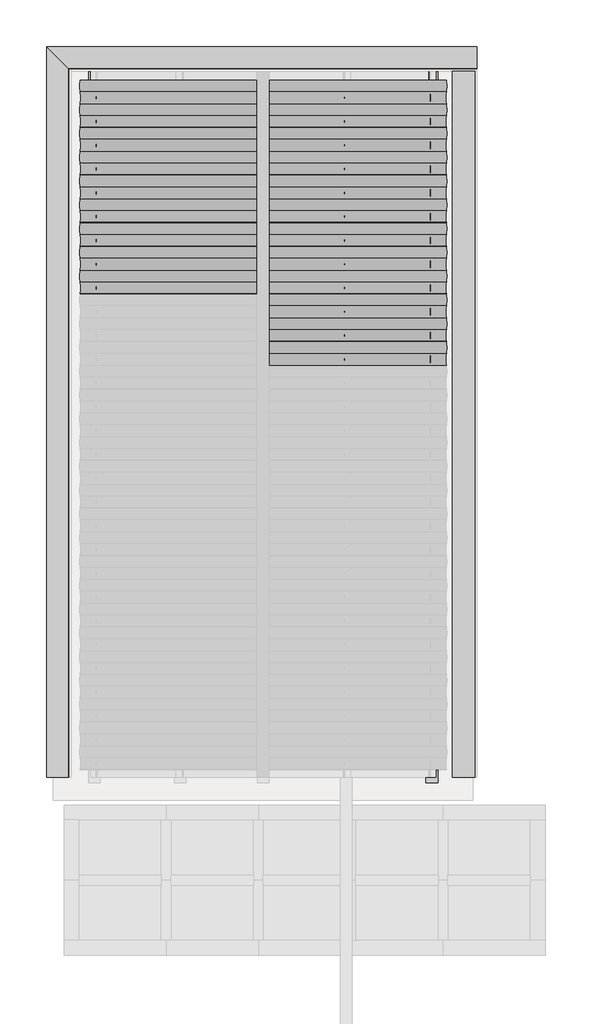
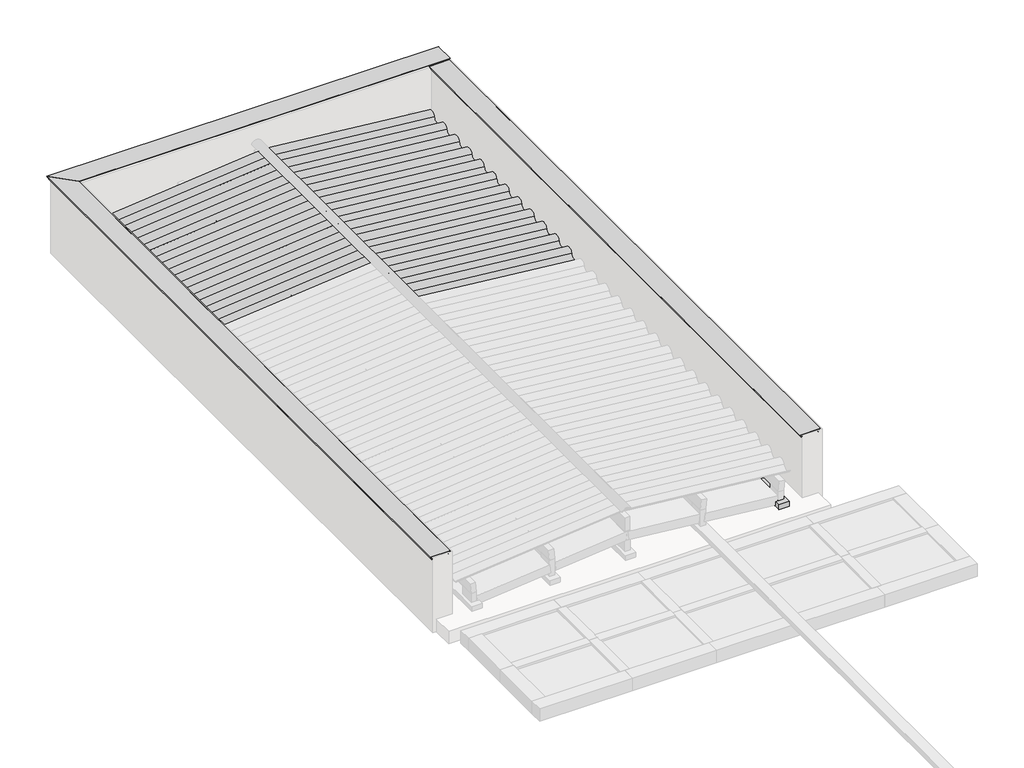
# One storey, part 3 of 3: 34 beams, 12 columns, 1 proxy.
"""IFC4 building model written with IfcOpenShell, lengths in millimetres."""

import ifcopenshell
import ifcopenshell.guid

model = None  # the IFC model being written
_history = None  # IfcOwnerHistory: only IFC2X3 demands one
_inside = {}  # id of a spatial element -> (the spatial element, [elements in it])
_under = {}  # id of a project, library or spatial element -> (it, [spatial elements below it])
_declared = {}  # id of a project -> (the project, [libraries it declares])
_typed = {}  # id of a type object -> (the type object, [elements of that type])
_made_of = {}  # id of a material, layer set ... -> (it, [elements and type objects made of it])


def new_model(schema):
    """Start an empty IFC model of exactly this schema.

    Asked for "IFC4X3", IfcOpenShell would pick the latest addendum, in which some entities
    have other attributes; the version numbers below select the first issue.
    IFC2X3 requires an IfcOwnerHistory on every rooted entity: one is made here for all.
    """
    global model, _history
    if schema == "IFC4X3":
        model = ifcopenshell.file(schema_version=(4, 3, 0, 0))
    else:
        model = ifcopenshell.file(schema=schema)
    _inside.clear()
    _under.clear()
    _declared.clear()
    _typed.clear()
    _made_of.clear()
    _history = None
    if model.schema == "IFC2X3":
        org = make("IfcOrganization", Name="unknown")
        user = make(
            "IfcPersonAndOrganization",
            ThePerson=make("IfcPerson", FamilyName="unknown"),
            TheOrganization=org,
        )
        app = make(
            "IfcApplication",
            ApplicationDeveloper=org,
            Version="unknown",
            ApplicationFullName="unknown",
            ApplicationIdentifier="unknown",
        )
        _history = make(
            "IfcOwnerHistory",
            OwningUser=user,
            OwningApplication=app,
            ChangeAction="ADDED",
            CreationDate=0,
        )
    return model


def make(cls, **values):
    """One entity of the class cls with the attributes given. An attribute that is None is left unset."""
    return model.create_entity(
        cls, **{name: value for name, value in values.items() if value is not None}
    )


def rooted(cls, **values):
    """An entity with a GlobalId (a new one), such as an element, a storey or a relation."""
    return make(cls, GlobalId=ifcopenshell.guid.new(), OwnerHistory=_history, **values)


def si_unit(unit_type, name, prefix=None):
    """IfcSIUnit, for example si_unit("LENGTHUNIT", "METRE", prefix="MILLI")."""
    return make("IfcSIUnit", UnitType=unit_type, Prefix=prefix, Name=name)


def assignment(units):
    """IfcUnitAssignment: the units of a project."""
    return None if units is None else make("IfcUnitAssignment", Units=units)


def point(xyz):
    """IfcCartesianPoint."""
    return None if xyz is None else make("IfcCartesianPoint", Coordinates=xyz)


def direction(xyz):
    """IfcDirection."""
    return None if xyz is None else make("IfcDirection", DirectionRatios=xyz)


def frame(location, z_axis=None, x_axis=None):
    """IfcAxis2Placement3D, a coordinate frame: its origin and axes. An axis left out is left unset."""
    return make(
        "IfcAxis2Placement3D",
        Location=point(location),
        Axis=direction(z_axis),
        RefDirection=direction(x_axis),
    )


def frame_2d(location, x_axis=None):
    """IfcAxis2Placement2D, a coordinate frame in the plane: its origin and x axis."""
    return make(
        "IfcAxis2Placement2D", Location=point(location), RefDirection=direction(x_axis)
    )


def origin():
    """The frame at (0, 0, 0) with its axes left unset."""
    return frame((0.0, 0.0, 0.0))


def place(relative_to, where):
    """IfcLocalPlacement: puts the frame where relative to a parent placement (None: the world)."""
    return make(
        "IfcLocalPlacement", PlacementRelTo=relative_to, RelativePlacement=where
    )


def context(
    kind, dimensions, precision=None, world=None, true_north=None, identifier=None
):
    """IfcGeometricRepresentationContext, for example the 3D "Model" context."""
    return make(
        "IfcGeometricRepresentationContext",
        ContextIdentifier=identifier,
        ContextType=kind,
        CoordinateSpaceDimension=dimensions,
        Precision=precision,
        WorldCoordinateSystem=world,
        TrueNorth=true_north,
    )


def project(units=None, contexts=None):
    """IfcProject with its units and contexts."""
    return rooted(
        "IfcProject",
        Name="project",
        RepresentationContexts=contexts,
        UnitsInContext=assignment(units),
    )


def spatial(cls, under=None, at=None, **own):
    """A site, building, storey or space (cls), placed at a placement, below another one or the project."""
    s = rooted(cls, ObjectPlacement=at, **own)
    if under is not None:
        _under.setdefault(under.id(), (under, []))[1].append(s)
    return s


def polyline(points):
    """IfcPolyline through the points."""
    return make("IfcPolyline", Points=[point(p) for p in points])


def circle_curve(where, radius):
    """IfcCircle in the frame where."""
    return make("IfcCircle", Position=where, Radius=radius)


def trimmed(basis, trim1, trim2, sense, master):
    """IfcTrimmedCurve: the piece of a basis curve between two trims."""
    return make(
        "IfcTrimmedCurve",
        BasisCurve=basis,
        Trim1=trim1,
        Trim2=trim2,
        SenseAgreement=sense,
        MasterRepresentation=master,
    )


def segment(curve, same_sense, transition):
    """IfcCompositeCurveSegment."""
    return make(
        "IfcCompositeCurveSegment",
        Transition=transition,
        SameSense=same_sense,
        ParentCurve=curve,
    )


def composite_curve(segments, self_intersect=None):
    """IfcCompositeCurve: segments joined end to end."""
    return make("IfcCompositeCurve", Segments=segments, SelfIntersect=self_intersect)


def outline(outer, holes=None, kind="AREA"):
    """IfcArbitraryClosedProfileDef: a profile drawn as a closed curve; with holes, ...WithVoids."""
    if holes is None:
        return make("IfcArbitraryClosedProfileDef", ProfileType=kind, OuterCurve=outer)
    return make(
        "IfcArbitraryProfileDefWithVoids",
        ProfileType=kind,
        OuterCurve=outer,
        InnerCurves=holes,
    )


def extrude(swept, where, along, depth):
    """IfcExtrudedAreaSolid: the profile swept, set in the frame where, extruded along a direction by depth."""
    return make(
        "IfcExtrudedAreaSolid",
        SweptArea=swept,
        Position=where,
        ExtrudedDirection=direction(along),
        Depth=depth,
    )


def faces_of(points, faces, orient=None, outer=None):
    """IfcFace entities. A face is a list of loops; a loop is a list of indices into points, from 0.

    orient and outer hold one flag for each loop. By default every Orientation is true, the
    first loop of a face is its IfcFaceOuterBound and the others are IfcFaceBound.
    """
    made = []
    for i, loops in enumerate(faces):
        bounds = []
        for j, loop in enumerate(loops):
            is_outer = j == 0 if outer is None else outer[i][j]
            bounds.append(
                make(
                    "IfcFaceOuterBound" if is_outer else "IfcFaceBound",
                    Bound=make("IfcPolyLoop", Polygon=[points[k] for k in loop]),
                    Orientation=True if orient is None else orient[i][j],
                )
            )
        made.append(make("IfcFace", Bounds=bounds))
    return made


def faceted_brep(points, faces, orient=None, outer=None, voids=None):
    """IfcFacetedBrep: a solid bounded by flat faces; with voids (closed shells), ...WithVoids."""
    shared = [point(p) for p in points]
    hull = make("IfcClosedShell", CfsFaces=faces_of(shared, faces, orient, outer))
    if voids is None:
        return make("IfcFacetedBrep", Outer=hull)
    return make(
        "IfcFacetedBrepWithVoids",
        Outer=hull,
        Voids=[
            make(cls, CfsFaces=faces_of(shared, fs, o, b)) for cls, fs, o, b in voids
        ],
    )


def shape(context_of_items, identifier, shape_type, items):
    """IfcShapeRepresentation: the items that make up one representation, for example the "Body"."""
    return make(
        "IfcShapeRepresentation",
        ContextOfItems=context_of_items,
        RepresentationIdentifier=identifier,
        RepresentationType=shape_type,
        Items=items,
    )


def source(mapping_origin, context_of_items, identifier, shape_type, items):
    """IfcRepresentationMap: a shape defined once, which mapped items show again and again."""
    return make(
        "IfcRepresentationMap",
        MappingOrigin=mapping_origin,
        MappedRepresentation=shape(context_of_items, identifier, shape_type, items),
    )


def transform(
    local_origin,
    x_axis=None,
    y_axis=None,
    z_axis=None,
    scale=None,
    scale2=None,
    scale3=None,
    uniform=True,
):
    """IfcCartesianTransformationOperator3D, or its non-uniform kind. x_axis, y_axis, z_axis: its Axis1, 2, 3."""
    if uniform:
        return make(
            "IfcCartesianTransformationOperator3D",
            Axis1=direction(x_axis),
            Axis2=direction(y_axis),
            LocalOrigin=point(local_origin),
            Scale=scale,
            Axis3=direction(z_axis),
        )
    return make(
        "IfcCartesianTransformationOperator3DnonUniform",
        Axis1=direction(x_axis),
        Axis2=direction(y_axis),
        LocalOrigin=point(local_origin),
        Scale=scale,
        Axis3=direction(z_axis),
        Scale2=scale2,
        Scale3=scale3,
    )


def mapped(mapping_source, mapping_target):
    """IfcMappedItem: shows the shape of a source again, moved by a transform."""
    return make(
        "IfcMappedItem", MappingSource=mapping_source, MappingTarget=mapping_target
    )


def made_of(thing, what):
    """Note that an element or type object is made of a material, layer set ...; save() writes the relation."""
    if what is not None:
        _made_of.setdefault(what.id(), (what, []))[1].append(thing)
    return thing


def element(
    cls,
    number,
    at=None,
    inside=None,
    cuts=None,
    type_object=None,
    material=None,
    context=None,
    identifier="Body",
    shape_type=None,
    held_by="IfcProductDefinitionShape",
    body=None,
    shapes=None,
    **own,
):
    """One element of the class cls, such as IfcWall. Its Tag is "e" and its number.

    at: its placement. inside: the storey or other place that contains it. cuts: it is an
    opening in that element (IfcRelVoidsElement). A single representation is given by context,
    identifier, shape_type and body (its items); several are given by shapes. held_by: the class
    of the entity that holds the representations. save() writes the other relations.
    """
    e = rooted(cls, Tag="e%d" % number, ObjectPlacement=at, **own)
    if body is not None:
        shapes = [shape(context, identifier, shape_type, body)]
    if shapes is not None:
        e.Representation = make(held_by, Representations=shapes)
    if inside is not None:
        _inside.setdefault(inside.id(), (inside, []))[1].append(e)
    if cuts is not None:
        rooted(
            "IfcRelVoidsElement", RelatingBuildingElement=cuts, RelatedOpeningElement=e
        )
    if type_object is not None:
        _typed.setdefault(type_object.id(), (type_object, []))[1].append(e)
    return made_of(e, material)


def aggregate(whole, parts):
    """IfcRelAggregates: a whole, such as a stair, and the parts it consists of."""
    return rooted("IfcRelAggregates", RelatingObject=whole, RelatedObjects=parts)


def save(model, path):
    """Write the relations noted so far, then the file.

    IfcRelAggregates (storeys below a building ...), IfcRelContainedInSpatialStructure (elements
    in a storey), IfcRelDefinesByType, IfcRelAssociatesMaterial and IfcRelDeclares: one each for
    every whole, place, type object, material and project.
    """
    for whole, parts in _under.values():
        aggregate(whole, parts)
    for where, things in _inside.values():
        rooted(
            "IfcRelContainedInSpatialStructure",
            RelatedElements=things,
            RelatingStructure=where,
        )
    for kind, things in _typed.values():
        rooted("IfcRelDefinesByType", RelatedObjects=things, RelatingType=kind)
    for what, things in _made_of.values():
        rooted("IfcRelAssociatesMaterial", RelatedObjects=things, RelatingMaterial=what)
    for by, libraries in _declared.values():
        rooted("IfcRelDeclares", RelatingContext=by, RelatedDefinitions=libraries)
    model.write(path)


def column_1cffec27(model_context):
    return source(origin(), model_context, "Body", "SweptSolid", [
        extrude(outline(polyline([(30.0, 80.0), (30.0, -80.0), (-30.0, -80.0), (-30.0, 80.0), (30.0, 80.0)])), frame((0.0, 0.0, 3110.0), z_axis=(0.0, 0.0, 1.0), x_axis=(1.0, 0.0, 0.0)), (0.0, 0.0, 1.0), 238.0),
    ])


def column_35730ad5(model_context):
    return source(origin(), model_context, "Body", "SweptSolid", [
        extrude(outline(polyline([(30.0, 80.0), (30.0, -80.0), (-30.0, -80.0), (-30.0, 80.0), (30.0, 80.0)])), frame((0.0, 0.0, 3110.0), z_axis=(0.0, 0.0, 1.0), x_axis=(1.0, 0.0, 0.0)), (0.0, 0.0, 1.0), 197.9),
    ])


def column_00c463e4(model_context):
    return source(origin(), model_context, "Body", "SweptSolid", [
        extrude(outline(polyline([(30.0, 80.0), (30.0, -80.0), (-30.0, -80.0), (-30.0, 80.0), (30.0, 80.0)])), frame((0.0, 0.0, 3110.0), z_axis=(0.0, 0.0, 1.0), x_axis=(1.0, 0.0, 0.0)), (0.0, 0.0, 1.0), 109.8),
    ])


model = new_model("IFC4")

# Units and contexts
model_context = context("Model", 3, world=origin())
ifc_project = project(units=[si_unit("LENGTHUNIT", "METRE", prefix="MILLI")], contexts=[model_context])

# Site, building, storey
site = spatial("IfcSite", under=ifc_project)
building = spatial("IfcBuilding", under=site)
storey = spatial("IfcBuildingStorey", under=building, Name="COB. GARAGEM", Elevation=3050.0)

# Beams
placement = place(None, origin())
element("IfcBeam", 1, ObjectType="Madeira de lei : Berço 6x12cm", at=placement, inside=storey, context=model_context, shape_type="SweptSolid", body=[
    extrude(outline(polyline([(-9620.281307, 6423.9300153), (-9500.281307, 6423.9300153), (-9500.281307, 4423.9300153), (-9620.281307, 4423.9300153), (-9620.281307, 6423.9300153)])), frame((0.0, 0.0, 3050.0), z_axis=(0.0, 0.0, 1.0), x_axis=(1.0, 0.0, 0.0)), (0.0, 0.0, 1.0), 60.0),
])
element("IfcBeam", 2, ObjectType="Madeira de lei : Berço 6x12cm", at=placement, inside=storey, context=model_context, shape_type="SweptSolid", body=[
    extrude(outline(polyline([(-9620.281307, 7083.9300153), (-9500.281307, 7083.9300153), (-9500.281307, 6423.9300153), (-9620.281307, 6423.9300153), (-9620.281307, 7083.9300153)])), frame((0.0, 0.0, 3050.0), z_axis=(0.0, 0.0, 1.0), x_axis=(1.0, 0.0, 0.0)), (0.0, 0.0, 1.0), 60.0),
])
element("IfcBeam", 3, ObjectType="Madeira de lei : Berço 6x12cm", at=placement, inside=storey, context=model_context, shape_type="SweptSolid", body=[
    extrude(outline(polyline([(-8767.0824227, 6423.9300153), (-8647.0824227, 6423.9300153), (-8647.0824227, 4423.9300153), (-8767.0824227, 4423.9300153), (-8767.0824227, 6423.9300153)])), frame((0.0, 0.0, 3050.0), z_axis=(0.0, 0.0, 1.0), x_axis=(1.0, 0.0, 0.0)), (0.0, 0.0, 1.0), 60.0),
])
element("IfcBeam", 4, ObjectType="Madeira de lei : Berço 6x12cm", at=placement, inside=storey, context=model_context, shape_type="SweptSolid", body=[
    extrude(outline(polyline([(-8767.0824227, 7083.9300153), (-8647.0824227, 7083.9300153), (-8647.0824227, 6423.9300153), (-8767.0824227, 6423.9300153), (-8767.0824227, 7083.9300153)])), frame((0.0, 0.0, 3050.0), z_axis=(0.0, 0.0, 1.0), x_axis=(1.0, 0.0, 0.0)), (0.0, 0.0, 1.0), 60.0),
])
element("IfcBeam", 5, ObjectType="Madeira de lei : Berço 6x12cm", at=placement, inside=storey, context=model_context, shape_type="SweptSolid", body=[
    extrude(outline(polyline([(-7884.0324227, 4423.9300153), (-7764.0324227, 4423.9300153), (-7764.0324227, 2423.9300153), (-7884.0324227, 2423.9300153), (-7884.0324227, 4423.9300153)])), frame((0.0, 0.0, 3050.0), z_axis=(0.0, 0.0, 1.0), x_axis=(1.0, 0.0, 0.0)), (0.0, 0.0, 1.0), 60.0),
])
element("IfcBeam", 6, ObjectType="Madeira de lei : Berço 6x12cm", at=placement, inside=storey, context=model_context, shape_type="SweptSolid", body=[
    extrude(outline(polyline([(-7884.0324227, 6423.9300153), (-7764.0324227, 6423.9300153), (-7764.0324227, 4423.9300153), (-7884.0324227, 4423.9300153), (-7884.0324227, 6423.9300153)])), frame((0.0, 0.0, 3050.0), z_axis=(0.0, 0.0, 1.0), x_axis=(1.0, 0.0, 0.0)), (0.0, 0.0, 1.0), 60.0),
])
element("IfcBeam", 7, ObjectType="Madeira de lei : Berço 6x12cm", at=placement, inside=storey, context=model_context, shape_type="SweptSolid", body=[
    extrude(outline(polyline([(-7884.0324227, 2423.9300153), (-7764.0324227, 2423.9300153), (-7764.0324227, 423.9300153), (-7884.0324227, 423.9300153), (-7884.0324227, 2423.9300153)])), frame((0.0, 0.0, 3050.0), z_axis=(0.0, 0.0, 1.0), x_axis=(1.0, 0.0, 0.0)), (0.0, 0.0, 1.0), 60.0),
])
element("IfcBeam", 8, ObjectType="Madeira de lei : Berço 6x12cm", at=placement, inside=storey, context=model_context, shape_type="SweptSolid", body=[
    extrude(outline(polyline([(-7884.0324227, 7083.9300153), (-7764.0324227, 7083.9300153), (-7764.0324227, 6423.9300153), (-7884.0324227, 6423.9300153), (-7884.0324227, 7083.9300153)])), frame((0.0, 0.0, 3050.0), z_axis=(0.0, 0.0, 1.0), x_axis=(1.0, 0.0, 0.0)), (0.0, 0.0, 1.0), 60.0),
])
element("IfcBeam", 9, ObjectType="Madeira de lei : Berço 6x12cm", at=placement, inside=storey, context=model_context, shape_type="SweptSolid", body=[
    extrude(outline(polyline([(-7884.0324227, 423.9300153), (-7764.0324227, 423.9300153), (-7764.0324227, -236.0699847), (-7884.0324227, -236.0699847), (-7884.0324227, 423.9300153)])), frame((0.0, 0.0, 3050.0), z_axis=(0.0, 0.0, 1.0), x_axis=(1.0, 0.0, 0.0)), (0.0, 0.0, 1.0), 60.0),
])
element("IfcBeam", 10, ObjectType="Madeira de lei : Berço 6x12cm", at=placement, inside=storey, context=model_context, shape_type="SweptSolid", body=[
    extrude(outline(polyline([(-10473.4801913, 6423.9300153), (-10353.4801913, 6423.9300153), (-10353.4801913, 4423.9300153), (-10473.4801913, 4423.9300153), (-10473.4801913, 6423.9300153)])), frame((0.0, 0.0, 3050.0), z_axis=(0.0, 0.0, 1.0), x_axis=(1.0, 0.0, 0.0)), (0.0, 0.0, 1.0), 60.0),
])
element("IfcBeam", 11, ObjectType="Madeira de lei : Berço 6x12cm", at=placement, inside=storey, context=model_context, shape_type="SweptSolid", body=[
    extrude(outline(polyline([(-10473.4801913, 7083.9300153), (-10353.4801913, 7083.9300153), (-10353.4801913, 6423.9300153), (-10473.4801913, 6423.9300153), (-10473.4801913, 7083.9300153)])), frame((0.0, 0.0, 3050.0), z_axis=(0.0, 0.0, 1.0), x_axis=(1.0, 0.0, 0.0)), (0.0, 0.0, 1.0), 60.0),
])
element("IfcBeam", 12, ObjectType="Madeira de lei : Berço 6x12cm", at=placement, inside=storey, context=model_context, shape_type="SweptSolid", body=[
    extrude(outline(polyline([(-11356.5301913, 6423.9300153), (-11236.5301913, 6423.9300153), (-11236.5301913, 4423.9300153), (-11356.5301913, 4423.9300153), (-11356.5301913, 6423.9300153)])), frame((0.0, 0.0, 3050.0), z_axis=(0.0, 0.0, 1.0), x_axis=(1.0, 0.0, 0.0)), (0.0, 0.0, 1.0), 60.0),
])
element("IfcBeam", 13, ObjectType="Madeira de lei : Berço 6x12cm", at=placement, inside=storey, context=model_context, shape_type="SweptSolid", body=[
    extrude(outline(polyline([(-11356.5301913, 7083.9300153), (-11236.5301913, 7083.9300153), (-11236.5301913, 6423.9300153), (-11356.5301913, 6423.9300153), (-11356.5301913, 7083.9300153)])), frame((0.0, 0.0, 3050.0), z_axis=(0.0, 0.0, 1.0), x_axis=(1.0, 0.0, 0.0)), (0.0, 0.0, 1.0), 60.0),
])
element("IfcBeam", 14, ObjectType="Telha Ondulada : Fibrocimento", at=placement, inside=storey, context=model_context, shape_type="SweptSolid", body=[
    extrude(outline(composite_curve([segment(trimmed(circle_curve(frame_2d((-58.7002979, -53.2060538)), 66.7939461), [point((-29.350149, 6.7939462))], [point((-29.350149, -113.2060538))], False, "CARTESIAN"), True, "CONTINUOUS"), segment(polyline([(-29.350149, -113.2060538), (-31.5472155, -108.7146288)]), True, "CONTINUOUS"), segment(trimmed(circle_curve(frame_2d((-58.7002979, -53.2060538)), 61.7939461), [point((-31.5472155, -108.7146288))], [point((-31.5472155, 2.3025211))], True, "CARTESIAN"), True, "CONTINUOUS"), segment(trimmed(circle_curve(frame_2d((0.0, 66.7939462)), 71.7939461), [point((-31.5472155, 2.3025211))], [point((-31.5472155, 131.2853712))], False, "CARTESIAN"), True, "CONTINUOUS"), segment(polyline([(-31.5472155, 131.2853712), (-29.350149, 126.7939462)]), True, "CONTINUOUS"), segment(trimmed(circle_curve(frame_2d((0.0, 66.7939462)), 66.7939461), [point((-29.350149, 126.7939462))], [point((-29.350149, 6.7939462))], True, "CARTESIAN"), True, "CONTINUOUS")], self_intersect=False)), frame((-11446.918865, 4918.826948, 3394.3067746), z_axis=(0.9950371902099892, 0.0, 0.09950371902099903), x_axis=(-0.09950371902099903, 0.0, 0.9950371902099892)), (0.0, 0.0, 1.0), 1886.8678854),
])
element("IfcBeam", 15, ObjectType="Telha Ondulada : Fibrocimento", at=placement, inside=storey, context=model_context, shape_type="SweptSolid", body=[
    extrude(outline(composite_curve([segment(trimmed(circle_curve(frame_2d((-58.7002979, -53.2060538)), 66.7939461), [point((-29.350149, 6.7939462))], [point((-29.350149, -113.2060538))], False, "CARTESIAN"), True, "CONTINUOUS"), segment(polyline([(-29.350149, -113.2060538), (-31.5472155, -108.7146288)]), True, "CONTINUOUS"), segment(trimmed(circle_curve(frame_2d((-58.7002979, -53.2060538)), 61.7939461), [point((-31.5472155, -108.7146288))], [point((-31.5472155, 2.3025211))], True, "CARTESIAN"), True, "CONTINUOUS"), segment(trimmed(circle_curve(frame_2d((0.0, 66.7939462)), 71.7939461), [point((-31.5472155, 2.3025211))], [point((-31.5472155, 131.2853712))], False, "CARTESIAN"), True, "CONTINUOUS"), segment(polyline([(-31.5472155, 131.2853712), (-29.350149, 126.7939462)]), True, "CONTINUOUS"), segment(trimmed(circle_curve(frame_2d((0.0, 66.7939462)), 66.7939461), [point((-29.350149, 126.7939462))], [point((-29.350149, 6.7939462))], True, "CARTESIAN"), True, "CONTINUOUS")], self_intersect=False)), frame((-11446.918865, 5163.326948, 3394.3067746), z_axis=(0.9950371902099892, 0.0, 0.09950371902099937), x_axis=(-0.09950371902099937, 0.0, 0.9950371902099892)), (0.0, 0.0, 1.0), 1886.8678854),
])
element("IfcBeam", 16, ObjectType="Telha Ondulada : Fibrocimento", at=placement, inside=storey, context=model_context, shape_type="SweptSolid", body=[
    extrude(outline(composite_curve([segment(trimmed(circle_curve(frame_2d((-58.7002979, -53.2060538)), 66.7939461), [point((-29.350149, 6.7939462))], [point((-29.350149, -113.2060538))], False, "CARTESIAN"), True, "CONTINUOUS"), segment(polyline([(-29.350149, -113.2060538), (-31.5472155, -108.7146288)]), True, "CONTINUOUS"), segment(trimmed(circle_curve(frame_2d((-58.7002979, -53.2060538)), 61.7939461), [point((-31.5472155, -108.7146288))], [point((-31.5472155, 2.3025211))], True, "CARTESIAN"), True, "CONTINUOUS"), segment(trimmed(circle_curve(frame_2d((0.0, 66.7939462)), 71.7939461), [point((-31.5472155, 2.3025211))], [point((-31.5472155, 131.2853712))], False, "CARTESIAN"), True, "CONTINUOUS"), segment(polyline([(-31.5472155, 131.2853712), (-29.350149, 126.7939462)]), True, "CONTINUOUS"), segment(trimmed(circle_curve(frame_2d((0.0, 66.7939462)), 66.7939461), [point((-29.350149, 126.7939462))], [point((-29.350149, 6.7939462))], True, "CARTESIAN"), True, "CONTINUOUS")], self_intersect=False)), frame((-11446.918865, 5407.826948, 3394.3067746), z_axis=(0.9950371902099892, 0.0, 0.09950371902099972), x_axis=(-0.09950371902099972, 0.0, 0.9950371902099892)), (0.0, 0.0, 1.0), 1886.8678854),
])
element("IfcBeam", 17, ObjectType="Telha Ondulada : Fibrocimento", at=placement, inside=storey, context=model_context, shape_type="SweptSolid", body=[
    extrude(outline(composite_curve([segment(trimmed(circle_curve(frame_2d((-58.7002979, -53.2060538)), 66.7939461), [point((-29.350149, 6.7939462))], [point((-29.350149, -113.2060538))], False, "CARTESIAN"), True, "CONTINUOUS"), segment(polyline([(-29.350149, -113.2060538), (-31.5472155, -108.7146288)]), True, "CONTINUOUS"), segment(trimmed(circle_curve(frame_2d((-58.7002979, -53.2060538)), 61.7939461), [point((-31.5472155, -108.7146288))], [point((-31.5472155, 2.3025211))], True, "CARTESIAN"), True, "CONTINUOUS"), segment(trimmed(circle_curve(frame_2d((0.0, 66.7939462)), 71.7939461), [point((-31.5472155, 2.3025211))], [point((-31.5472155, 131.2853712))], False, "CARTESIAN"), True, "CONTINUOUS"), segment(polyline([(-31.5472155, 131.2853712), (-29.350149, 126.7939462)]), True, "CONTINUOUS"), segment(trimmed(circle_curve(frame_2d((0.0, 66.7939462)), 66.7939461), [point((-29.350149, 126.7939462))], [point((-29.350149, 6.7939462))], True, "CARTESIAN"), True, "CONTINUOUS")], self_intersect=False)), frame((-11446.918865, 5652.326948, 3394.3067746), z_axis=(0.9950371902099892, 0.0, 0.09950371902099954), x_axis=(-0.09950371902099954, 0.0, 0.9950371902099892)), (0.0, 0.0, 1.0), 1886.8678854),
])
element("IfcBeam", 18, ObjectType="Telha Ondulada : Fibrocimento", at=placement, inside=storey, context=model_context, shape_type="SweptSolid", body=[
    extrude(outline(composite_curve([segment(trimmed(circle_curve(frame_2d((-58.7002979, -53.2060538)), 66.7939461), [point((-29.350149, 6.7939462))], [point((-29.350149, -113.2060538))], False, "CARTESIAN"), True, "CONTINUOUS"), segment(polyline([(-29.350149, -113.2060538), (-31.5472155, -108.7146288)]), True, "CONTINUOUS"), segment(trimmed(circle_curve(frame_2d((-58.7002979, -53.2060538)), 61.7939461), [point((-31.5472155, -108.7146288))], [point((-31.5472155, 2.3025211))], True, "CARTESIAN"), True, "CONTINUOUS"), segment(trimmed(circle_curve(frame_2d((0.0, 66.7939462)), 71.7939461), [point((-31.5472155, 2.3025211))], [point((-31.5472155, 131.2853712))], False, "CARTESIAN"), True, "CONTINUOUS"), segment(polyline([(-31.5472155, 131.2853712), (-29.350149, 126.7939462)]), True, "CONTINUOUS"), segment(trimmed(circle_curve(frame_2d((0.0, 66.7939462)), 66.7939461), [point((-29.350149, 126.7939462))], [point((-29.350149, 6.7939462))], True, "CARTESIAN"), True, "CONTINUOUS")], self_intersect=False)), frame((-11446.918865, 5896.826948, 3394.3067746), z_axis=(0.9950371902099892, 0.0, 0.09950371902099932), x_axis=(-0.09950371902099932, 0.0, 0.9950371902099892)), (0.0, 0.0, 1.0), 1886.8678854),
])
element("IfcBeam", 19, ObjectType="Telha Ondulada : Fibrocimento", at=placement, inside=storey, context=model_context, shape_type="SweptSolid", body=[
    extrude(outline(composite_curve([segment(trimmed(circle_curve(frame_2d((-58.7002979, -53.2060538)), 66.7939461), [point((-29.350149, 6.7939462))], [point((-29.350149, -113.2060538))], False, "CARTESIAN"), True, "CONTINUOUS"), segment(polyline([(-29.350149, -113.2060538), (-31.5472155, -108.7146288)]), True, "CONTINUOUS"), segment(trimmed(circle_curve(frame_2d((-58.7002979, -53.2060538)), 61.7939461), [point((-31.5472155, -108.7146288))], [point((-31.5472155, 2.3025211))], True, "CARTESIAN"), True, "CONTINUOUS"), segment(trimmed(circle_curve(frame_2d((0.0, 66.7939462)), 71.7939461), [point((-31.5472155, 2.3025211))], [point((-31.5472155, 131.2853712))], False, "CARTESIAN"), True, "CONTINUOUS"), segment(polyline([(-31.5472155, 131.2853712), (-29.350149, 126.7939462)]), True, "CONTINUOUS"), segment(trimmed(circle_curve(frame_2d((0.0, 66.7939462)), 66.7939461), [point((-29.350149, 126.7939462))], [point((-29.350149, 6.7939462))], True, "CARTESIAN"), True, "CONTINUOUS")], self_intersect=False)), frame((-11446.918865, 6141.326948, 3394.3067746), z_axis=(0.9950371902099892, 0.0, 0.09950371902099943), x_axis=(-0.09950371902099943, 0.0, 0.9950371902099892)), (0.0, 0.0, 1.0), 1886.8678854),
])
element("IfcBeam", 20, ObjectType="Telha Ondulada : Fibrocimento", at=placement, inside=storey, context=model_context, shape_type="SweptSolid", body=[
    extrude(outline(composite_curve([segment(trimmed(circle_curve(frame_2d((-58.7002979, -53.2060538)), 66.7939461), [point((-29.350149, 6.7939462))], [point((-29.350149, -113.2060538))], False, "CARTESIAN"), True, "CONTINUOUS"), segment(polyline([(-29.350149, -113.2060538), (-31.5472155, -108.7146288)]), True, "CONTINUOUS"), segment(trimmed(circle_curve(frame_2d((-58.7002979, -53.2060538)), 61.7939461), [point((-31.5472155, -108.7146288))], [point((-31.5472155, 2.3025211))], True, "CARTESIAN"), True, "CONTINUOUS"), segment(trimmed(circle_curve(frame_2d((0.0, 66.7939462)), 71.7939461), [point((-31.5472155, 2.3025211))], [point((-31.5472155, 131.2853712))], False, "CARTESIAN"), True, "CONTINUOUS"), segment(polyline([(-31.5472155, 131.2853712), (-29.350149, 126.7939462)]), True, "CONTINUOUS"), segment(trimmed(circle_curve(frame_2d((0.0, 66.7939462)), 66.7939461), [point((-29.350149, 126.7939462))], [point((-29.350149, 6.7939462))], True, "CARTESIAN"), True, "CONTINUOUS")], self_intersect=False)), frame((-11446.918865, 6385.826948, 3394.3067746), z_axis=(0.9950371902099892, 0.0, 0.09950371902099919), x_axis=(-0.09950371902099919, 0.0, 0.9950371902099892)), (0.0, 0.0, 1.0), 1886.8678854),
])
element("IfcBeam", 21, ObjectType="Telha Ondulada : Fibrocimento", at=placement, inside=storey, context=model_context, shape_type="SweptSolid", body=[
    extrude(outline(composite_curve([segment(trimmed(circle_curve(frame_2d((-58.7002979, -53.2060538)), 66.7939461), [point((-29.350149, 6.7939462))], [point((-29.350149, -113.2060538))], False, "CARTESIAN"), True, "CONTINUOUS"), segment(polyline([(-29.350149, -113.2060538), (-31.5472155, -108.7146288)]), True, "CONTINUOUS"), segment(trimmed(circle_curve(frame_2d((-58.7002979, -53.2060538)), 61.7939461), [point((-31.5472155, -108.7146288))], [point((-31.5472155, 2.3025211))], True, "CARTESIAN"), True, "CONTINUOUS"), segment(trimmed(circle_curve(frame_2d((0.0, 66.7939462)), 71.7939461), [point((-31.5472155, 2.3025211))], [point((-31.5472155, 131.2853712))], False, "CARTESIAN"), True, "CONTINUOUS"), segment(polyline([(-31.5472155, 131.2853712), (-29.350149, 126.7939462)]), True, "CONTINUOUS"), segment(trimmed(circle_curve(frame_2d((0.0, 66.7939462)), 66.7939461), [point((-29.350149, 126.7939462))], [point((-29.350149, 6.7939462))], True, "CARTESIAN"), True, "CONTINUOUS")], self_intersect=False)), frame((-11446.918865, 6630.326948, 3394.3067746), z_axis=(0.9950371902099892, 0.0, 0.09950371902099925), x_axis=(-0.09950371902099925, 0.0, 0.9950371902099892)), (0.0, 0.0, 1.0), 1886.8678854),
])
element("IfcBeam", 22, ObjectType="Telha Ondulada : Fibrocimento", at=placement, inside=storey, context=model_context, shape_type="SweptSolid", body=[
    extrude(outline(composite_curve([segment(trimmed(circle_curve(frame_2d((-58.7002979, -53.2060538)), 66.7939461), [point((-29.350149, 6.7939462))], [point((-29.350149, -113.2060538))], False, "CARTESIAN"), True, "CONTINUOUS"), segment(polyline([(-29.350149, -113.2060538), (-31.5472155, -108.7146288)]), True, "CONTINUOUS"), segment(trimmed(circle_curve(frame_2d((-58.7002979, -53.2060538)), 61.7939461), [point((-31.5472155, -108.7146288))], [point((-31.5472155, 2.3025211))], True, "CARTESIAN"), True, "CONTINUOUS"), segment(trimmed(circle_curve(frame_2d((0.0, 66.7939462)), 71.7939461), [point((-31.5472155, 2.3025211))], [point((-31.5472155, 131.2853712))], False, "CARTESIAN"), True, "CONTINUOUS"), segment(polyline([(-31.5472155, 131.2853712), (-29.350149, 126.7939462)]), True, "CONTINUOUS"), segment(trimmed(circle_curve(frame_2d((0.0, 66.7939462)), 66.7939461), [point((-29.350149, 126.7939462))], [point((-29.350149, 6.7939462))], True, "CARTESIAN"), True, "CONTINUOUS")], self_intersect=False)), frame((-11446.918865, 6874.826948, 3394.3067746), z_axis=(0.9950371902099892, 0.0, 0.09950371902099937), x_axis=(-0.09950371902099937, 0.0, 0.9950371902099892)), (0.0, 0.0, 1.0), 1886.8678854),
])
element("IfcBeam", 23, ObjectType="Telha Ondulada : Fibrocimento", at=placement, inside=storey, context=model_context, shape_type="SweptSolid", body=[
    extrude(outline(composite_curve([segment(trimmed(circle_curve(frame_2d((0.0, 66.7939462)), 66.7939461), [point((29.350149, 6.7939462))], [point((29.350149, 126.7939462))], True, "CARTESIAN"), True, "CONTINUOUS"), segment(polyline([(29.350149, 126.7939462), (31.5472155, 131.2853712)]), True, "CONTINUOUS"), segment(trimmed(circle_curve(frame_2d((0.0, 66.7939462)), 71.7939461), [point((31.5472155, 131.2853712))], [point((31.5472155, 2.3025211))], False, "CARTESIAN"), True, "CONTINUOUS"), segment(trimmed(circle_curve(frame_2d((58.7002979, -53.2060538)), 61.7939461), [point((31.5472155, 2.3025211))], [point((31.5472155, -108.7146288))], True, "CARTESIAN"), True, "CONTINUOUS"), segment(polyline([(31.5472155, -108.7146288), (29.350149, -113.2060538)]), True, "CONTINUOUS"), segment(trimmed(circle_curve(frame_2d((58.7002979, -53.2060538)), 66.7939461), [point((29.350149, -113.2060538))], [point((29.350149, 6.7939462))], False, "CARTESIAN"), True, "CONTINUOUS")], self_intersect=False)), frame((-7673.6437489, 4185.326948, 3394.3067746), z_axis=(-0.9950371902099892, 0.0, 0.09950371902099979), x_axis=(-0.09950371902099979, 0.0, -0.9950371902099892)), (0.0, 0.0, 1.0), 1886.8678854),
])
element("IfcBeam", 24, ObjectType="Telha Ondulada : Fibrocimento", at=placement, inside=storey, context=model_context, shape_type="SweptSolid", body=[
    extrude(outline(composite_curve([segment(trimmed(circle_curve(frame_2d((0.0, 66.7939462)), 66.7939461), [point((29.350149, 6.7939462))], [point((29.350149, 126.7939462))], True, "CARTESIAN"), True, "CONTINUOUS"), segment(polyline([(29.350149, 126.7939462), (31.5472155, 131.2853712)]), True, "CONTINUOUS"), segment(trimmed(circle_curve(frame_2d((0.0, 66.7939462)), 71.7939461), [point((31.5472155, 131.2853712))], [point((31.5472155, 2.3025211))], False, "CARTESIAN"), True, "CONTINUOUS"), segment(trimmed(circle_curve(frame_2d((58.7002979, -53.2060538)), 61.7939461), [point((31.5472155, 2.3025211))], [point((31.5472155, -108.7146288))], True, "CARTESIAN"), True, "CONTINUOUS"), segment(polyline([(31.5472155, -108.7146288), (29.350149, -113.2060538)]), True, "CONTINUOUS"), segment(trimmed(circle_curve(frame_2d((58.7002979, -53.2060538)), 66.7939461), [point((29.350149, -113.2060538))], [point((29.350149, 6.7939462))], False, "CARTESIAN"), True, "CONTINUOUS")], self_intersect=False)), frame((-7673.6437489, 4429.826948, 3394.3067746), z_axis=(-0.9950371902099892, 0.0, 0.09950371902099979), x_axis=(-0.09950371902099979, 0.0, -0.9950371902099892)), (0.0, 0.0, 1.0), 1886.8678854),
])
element("IfcBeam", 25, ObjectType="Telha Ondulada : Fibrocimento", at=placement, inside=storey, context=model_context, shape_type="SweptSolid", body=[
    extrude(outline(composite_curve([segment(trimmed(circle_curve(frame_2d((0.0, 66.7939462)), 66.7939461), [point((29.350149, 6.7939462))], [point((29.350149, 126.7939462))], True, "CARTESIAN"), True, "CONTINUOUS"), segment(polyline([(29.350149, 126.7939462), (31.5472155, 131.2853712)]), True, "CONTINUOUS"), segment(trimmed(circle_curve(frame_2d((0.0, 66.7939462)), 71.7939461), [point((31.5472155, 131.2853712))], [point((31.5472155, 2.3025211))], False, "CARTESIAN"), True, "CONTINUOUS"), segment(trimmed(circle_curve(frame_2d((58.7002979, -53.2060538)), 61.7939461), [point((31.5472155, 2.3025211))], [point((31.5472155, -108.7146288))], True, "CARTESIAN"), True, "CONTINUOUS"), segment(polyline([(31.5472155, -108.7146288), (29.350149, -113.2060538)]), True, "CONTINUOUS"), segment(trimmed(circle_curve(frame_2d((58.7002979, -53.2060538)), 66.7939461), [point((29.350149, -113.2060538))], [point((29.350149, 6.7939462))], False, "CARTESIAN"), True, "CONTINUOUS")], self_intersect=False)), frame((-7673.6437489, 4674.326948, 3394.3067746), z_axis=(-0.9950371902099892, 0.0, 0.09950371902099979), x_axis=(-0.09950371902099979, 0.0, -0.9950371902099892)), (0.0, 0.0, 1.0), 1886.8678854),
])
element("IfcBeam", 26, ObjectType="Telha Ondulada : Fibrocimento", at=placement, inside=storey, context=model_context, shape_type="SweptSolid", body=[
    extrude(outline(composite_curve([segment(trimmed(circle_curve(frame_2d((0.0, 66.7939462)), 66.7939461), [point((29.350149, 6.7939462))], [point((29.350149, 126.7939462))], True, "CARTESIAN"), True, "CONTINUOUS"), segment(polyline([(29.350149, 126.7939462), (31.5472155, 131.2853712)]), True, "CONTINUOUS"), segment(trimmed(circle_curve(frame_2d((0.0, 66.7939462)), 71.7939461), [point((31.5472155, 131.2853712))], [point((31.5472155, 2.3025211))], False, "CARTESIAN"), True, "CONTINUOUS"), segment(trimmed(circle_curve(frame_2d((58.7002979, -53.2060538)), 61.7939461), [point((31.5472155, 2.3025211))], [point((31.5472155, -108.7146288))], True, "CARTESIAN"), True, "CONTINUOUS"), segment(polyline([(31.5472155, -108.7146288), (29.350149, -113.2060538)]), True, "CONTINUOUS"), segment(trimmed(circle_curve(frame_2d((58.7002979, -53.2060538)), 66.7939461), [point((29.350149, -113.2060538))], [point((29.350149, 6.7939462))], False, "CARTESIAN"), True, "CONTINUOUS")], self_intersect=False)), frame((-7673.6437489, 4918.826948, 3394.3067746), z_axis=(-0.9950371902099892, 0.0, 0.09950371902099979), x_axis=(-0.09950371902099979, 0.0, -0.9950371902099892)), (0.0, 0.0, 1.0), 1886.8678854),
])
element("IfcBeam", 27, ObjectType="Telha Ondulada : Fibrocimento", at=placement, inside=storey, context=model_context, shape_type="SweptSolid", body=[
    extrude(outline(composite_curve([segment(trimmed(circle_curve(frame_2d((0.0, 66.7939462)), 66.7939461), [point((29.350149, 6.7939462))], [point((29.350149, 126.7939462))], True, "CARTESIAN"), True, "CONTINUOUS"), segment(polyline([(29.350149, 126.7939462), (31.5472155, 131.2853712)]), True, "CONTINUOUS"), segment(trimmed(circle_curve(frame_2d((0.0, 66.7939462)), 71.7939461), [point((31.5472155, 131.2853712))], [point((31.5472155, 2.3025211))], False, "CARTESIAN"), True, "CONTINUOUS"), segment(trimmed(circle_curve(frame_2d((58.7002979, -53.2060538)), 61.7939461), [point((31.5472155, 2.3025211))], [point((31.5472155, -108.7146288))], True, "CARTESIAN"), True, "CONTINUOUS"), segment(polyline([(31.5472155, -108.7146288), (29.350149, -113.2060538)]), True, "CONTINUOUS"), segment(trimmed(circle_curve(frame_2d((58.7002979, -53.2060538)), 66.7939461), [point((29.350149, -113.2060538))], [point((29.350149, 6.7939462))], False, "CARTESIAN"), True, "CONTINUOUS")], self_intersect=False)), frame((-7673.6437489, 5163.326948, 3394.3067746), z_axis=(-0.9950371902099892, 0.0, 0.09950371902099979), x_axis=(-0.09950371902099979, 0.0, -0.9950371902099892)), (0.0, 0.0, 1.0), 1886.8678854),
])
element("IfcBeam", 28, ObjectType="Telha Ondulada : Fibrocimento", at=placement, inside=storey, context=model_context, shape_type="SweptSolid", body=[
    extrude(outline(composite_curve([segment(trimmed(circle_curve(frame_2d((0.0, 66.7939462)), 66.7939461), [point((29.350149, 6.7939462))], [point((29.350149, 126.7939462))], True, "CARTESIAN"), True, "CONTINUOUS"), segment(polyline([(29.350149, 126.7939462), (31.5472155, 131.2853712)]), True, "CONTINUOUS"), segment(trimmed(circle_curve(frame_2d((0.0, 66.7939462)), 71.7939461), [point((31.5472155, 131.2853712))], [point((31.5472155, 2.3025211))], False, "CARTESIAN"), True, "CONTINUOUS"), segment(trimmed(circle_curve(frame_2d((58.7002979, -53.2060538)), 61.7939461), [point((31.5472155, 2.3025211))], [point((31.5472155, -108.7146288))], True, "CARTESIAN"), True, "CONTINUOUS"), segment(polyline([(31.5472155, -108.7146288), (29.350149, -113.2060538)]), True, "CONTINUOUS"), segment(trimmed(circle_curve(frame_2d((58.7002979, -53.2060538)), 66.7939461), [point((29.350149, -113.2060538))], [point((29.350149, 6.7939462))], False, "CARTESIAN"), True, "CONTINUOUS")], self_intersect=False)), frame((-7673.6437489, 5407.826948, 3394.3067746), z_axis=(-0.9950371902099892, 0.0, 0.09950371902099979), x_axis=(-0.09950371902099979, 0.0, -0.9950371902099892)), (0.0, 0.0, 1.0), 1886.8678854),
])
element("IfcBeam", 29, ObjectType="Telha Ondulada : Fibrocimento", at=placement, inside=storey, context=model_context, shape_type="SweptSolid", body=[
    extrude(outline(composite_curve([segment(trimmed(circle_curve(frame_2d((0.0, 66.7939462)), 66.7939461), [point((29.350149, 6.7939462))], [point((29.350149, 126.7939462))], True, "CARTESIAN"), True, "CONTINUOUS"), segment(polyline([(29.350149, 126.7939462), (31.5472155, 131.2853712)]), True, "CONTINUOUS"), segment(trimmed(circle_curve(frame_2d((0.0, 66.7939462)), 71.7939461), [point((31.5472155, 131.2853712))], [point((31.5472155, 2.3025211))], False, "CARTESIAN"), True, "CONTINUOUS"), segment(trimmed(circle_curve(frame_2d((58.7002979, -53.2060538)), 61.7939461), [point((31.5472155, 2.3025211))], [point((31.5472155, -108.7146288))], True, "CARTESIAN"), True, "CONTINUOUS"), segment(polyline([(31.5472155, -108.7146288), (29.350149, -113.2060538)]), True, "CONTINUOUS"), segment(trimmed(circle_curve(frame_2d((58.7002979, -53.2060538)), 66.7939461), [point((29.350149, -113.2060538))], [point((29.350149, 6.7939462))], False, "CARTESIAN"), True, "CONTINUOUS")], self_intersect=False)), frame((-7673.6437489, 5652.326948, 3394.3067746), z_axis=(-0.9950371902099892, 0.0, 0.09950371902099979), x_axis=(-0.09950371902099979, 0.0, -0.9950371902099892)), (0.0, 0.0, 1.0), 1886.8678854),
])
element("IfcBeam", 30, ObjectType="Telha Ondulada : Fibrocimento", at=placement, inside=storey, context=model_context, shape_type="SweptSolid", body=[
    extrude(outline(composite_curve([segment(trimmed(circle_curve(frame_2d((0.0, 66.7939462)), 66.7939461), [point((29.350149, 6.7939462))], [point((29.350149, 126.7939462))], True, "CARTESIAN"), True, "CONTINUOUS"), segment(polyline([(29.350149, 126.7939462), (31.5472155, 131.2853712)]), True, "CONTINUOUS"), segment(trimmed(circle_curve(frame_2d((0.0, 66.7939462)), 71.7939461), [point((31.5472155, 131.2853712))], [point((31.5472155, 2.3025211))], False, "CARTESIAN"), True, "CONTINUOUS"), segment(trimmed(circle_curve(frame_2d((58.7002979, -53.2060538)), 61.7939461), [point((31.5472155, 2.3025211))], [point((31.5472155, -108.7146288))], True, "CARTESIAN"), True, "CONTINUOUS"), segment(polyline([(31.5472155, -108.7146288), (29.350149, -113.2060538)]), True, "CONTINUOUS"), segment(trimmed(circle_curve(frame_2d((58.7002979, -53.2060538)), 66.7939461), [point((29.350149, -113.2060538))], [point((29.350149, 6.7939462))], False, "CARTESIAN"), True, "CONTINUOUS")], self_intersect=False)), frame((-7673.6437489, 5896.826948, 3394.3067746), z_axis=(-0.9950371902099892, 0.0, 0.09950371902099979), x_axis=(-0.09950371902099979, 0.0, -0.9950371902099892)), (0.0, 0.0, 1.0), 1886.8678854),
])
element("IfcBeam", 31, ObjectType="Telha Ondulada : Fibrocimento", at=placement, inside=storey, context=model_context, shape_type="SweptSolid", body=[
    extrude(outline(composite_curve([segment(trimmed(circle_curve(frame_2d((0.0, 66.7939462)), 66.7939461), [point((29.350149, 6.7939462))], [point((29.350149, 126.7939462))], True, "CARTESIAN"), True, "CONTINUOUS"), segment(polyline([(29.350149, 126.7939462), (31.5472155, 131.2853712)]), True, "CONTINUOUS"), segment(trimmed(circle_curve(frame_2d((0.0, 66.7939462)), 71.7939461), [point((31.5472155, 131.2853712))], [point((31.5472155, 2.3025211))], False, "CARTESIAN"), True, "CONTINUOUS"), segment(trimmed(circle_curve(frame_2d((58.7002979, -53.2060538)), 61.7939461), [point((31.5472155, 2.3025211))], [point((31.5472155, -108.7146288))], True, "CARTESIAN"), True, "CONTINUOUS"), segment(polyline([(31.5472155, -108.7146288), (29.350149, -113.2060538)]), True, "CONTINUOUS"), segment(trimmed(circle_curve(frame_2d((58.7002979, -53.2060538)), 66.7939461), [point((29.350149, -113.2060538))], [point((29.350149, 6.7939462))], False, "CARTESIAN"), True, "CONTINUOUS")], self_intersect=False)), frame((-7673.6437489, 6141.326948, 3394.3067746), z_axis=(-0.9950371902099892, 0.0, 0.09950371902099979), x_axis=(-0.09950371902099979, 0.0, -0.9950371902099892)), (0.0, 0.0, 1.0), 1886.8678854),
])
element("IfcBeam", 32, ObjectType="Telha Ondulada : Fibrocimento", at=placement, inside=storey, context=model_context, shape_type="SweptSolid", body=[
    extrude(outline(composite_curve([segment(trimmed(circle_curve(frame_2d((0.0, 66.7939462)), 66.7939461), [point((29.350149, 6.7939462))], [point((29.350149, 126.7939462))], True, "CARTESIAN"), True, "CONTINUOUS"), segment(polyline([(29.350149, 126.7939462), (31.5472155, 131.2853712)]), True, "CONTINUOUS"), segment(trimmed(circle_curve(frame_2d((0.0, 66.7939462)), 71.7939461), [point((31.5472155, 131.2853712))], [point((31.5472155, 2.3025211))], False, "CARTESIAN"), True, "CONTINUOUS"), segment(trimmed(circle_curve(frame_2d((58.7002979, -53.2060538)), 61.7939461), [point((31.5472155, 2.3025211))], [point((31.5472155, -108.7146288))], True, "CARTESIAN"), True, "CONTINUOUS"), segment(polyline([(31.5472155, -108.7146288), (29.350149, -113.2060538)]), True, "CONTINUOUS"), segment(trimmed(circle_curve(frame_2d((58.7002979, -53.2060538)), 66.7939461), [point((29.350149, -113.2060538))], [point((29.350149, 6.7939462))], False, "CARTESIAN"), True, "CONTINUOUS")], self_intersect=False)), frame((-7673.6437489, 6385.826948, 3394.3067746), z_axis=(-0.9950371902099892, 0.0, 0.09950371902099979), x_axis=(-0.09950371902099979, 0.0, -0.9950371902099892)), (0.0, 0.0, 1.0), 1886.8678854),
])
element("IfcBeam", 33, ObjectType="Telha Ondulada : Fibrocimento", at=placement, inside=storey, context=model_context, shape_type="SweptSolid", body=[
    extrude(outline(composite_curve([segment(trimmed(circle_curve(frame_2d((0.0, 66.7939462)), 66.7939461), [point((29.350149, 6.7939462))], [point((29.350149, 126.7939462))], True, "CARTESIAN"), True, "CONTINUOUS"), segment(polyline([(29.350149, 126.7939462), (31.5472155, 131.2853712)]), True, "CONTINUOUS"), segment(trimmed(circle_curve(frame_2d((0.0, 66.7939462)), 71.7939461), [point((31.5472155, 131.2853712))], [point((31.5472155, 2.3025211))], False, "CARTESIAN"), True, "CONTINUOUS"), segment(trimmed(circle_curve(frame_2d((58.7002979, -53.2060538)), 61.7939461), [point((31.5472155, 2.3025211))], [point((31.5472155, -108.7146288))], True, "CARTESIAN"), True, "CONTINUOUS"), segment(polyline([(31.5472155, -108.7146288), (29.350149, -113.2060538)]), True, "CONTINUOUS"), segment(trimmed(circle_curve(frame_2d((58.7002979, -53.2060538)), 66.7939461), [point((29.350149, -113.2060538))], [point((29.350149, 6.7939462))], False, "CARTESIAN"), True, "CONTINUOUS")], self_intersect=False)), frame((-7673.6437489, 6630.326948, 3394.3067746), z_axis=(-0.9950371902099892, 0.0, 0.09950371902099979), x_axis=(-0.09950371902099979, 0.0, -0.9950371902099892)), (0.0, 0.0, 1.0), 1886.8678854),
])
element("IfcBeam", 34, ObjectType="Telha Ondulada : Fibrocimento", at=placement, inside=storey, context=model_context, shape_type="SweptSolid", body=[
    extrude(outline(composite_curve([segment(trimmed(circle_curve(frame_2d((0.0, 66.7939462)), 66.7939461), [point((29.350149, 6.7939462))], [point((29.350149, 126.7939462))], True, "CARTESIAN"), True, "CONTINUOUS"), segment(polyline([(29.350149, 126.7939462), (31.5472155, 131.2853712)]), True, "CONTINUOUS"), segment(trimmed(circle_curve(frame_2d((0.0, 66.7939462)), 71.7939461), [point((31.5472155, 131.2853712))], [point((31.5472155, 2.3025211))], False, "CARTESIAN"), True, "CONTINUOUS"), segment(trimmed(circle_curve(frame_2d((58.7002979, -53.2060538)), 61.7939461), [point((31.5472155, 2.3025211))], [point((31.5472155, -108.7146288))], True, "CARTESIAN"), True, "CONTINUOUS"), segment(polyline([(31.5472155, -108.7146288), (29.350149, -113.2060538)]), True, "CONTINUOUS"), segment(trimmed(circle_curve(frame_2d((58.7002979, -53.2060538)), 66.7939461), [point((29.350149, -113.2060538))], [point((29.350149, 6.7939462))], False, "CARTESIAN"), True, "CONTINUOUS")], self_intersect=False)), frame((-7673.6437489, 6874.826948, 3394.3067746), z_axis=(-0.9950371902099892, 0.0, 0.09950371902099979), x_axis=(-0.09950371902099979, 0.0, -0.9950371902099892)), (0.0, 0.0, 1.0), 1886.8678854),
])

# Proxy
element("IfcBuildingElementProxy", 35, Name=".CC_RUFO_PINGADEIRA_22 cm", ObjectType=".CC_RUFO_PINGADEIRA_22 cm", at=placement, inside=storey, context=model_context, shape_type="Brep", body=[
    faceted_brep([(-7593.5024445, -175.5699847, 3776.6820963), (-7586.4313766, -175.5699847, 3783.7531641), (-7586.4313766, -175.5699847, 3786.5815912), (-7593.0054581, -175.5699847, 3780.0075098), (-7608.952748, -175.5699847, 3810.0), (-7385.6098659, -175.5699847, 3810.0), (-7401.5571559, -175.5699847, 3780.0075098), (-7408.1312373, -175.5699847, 3786.5815912), (-7408.1312373, -175.5699847, 3783.7531641), (-7401.0601695, -175.5699847, 3776.6820963), (-7382.281307, -175.5699847, 3812.0), (-7612.281307, -175.5699847, 3812.0), (-7593.5024445, 7082.4300153, 3776.6820963), (-7612.281307, 7082.4300153, 3812.0), (-7382.281307, 7082.4300153, 3812.0), (-7401.0601695, 7082.4300153, 3776.6820963), (-7408.1312373, 7082.4300153, 3783.7531641), (-7408.1312373, 7082.4300153, 3786.5815912), (-7401.5571559, 7082.4300153, 3780.0075098), (-7385.6098659, 7082.4300153, 3810.0), (-7608.952748, 7082.4300153, 3810.0), (-7593.0054581, 7082.4300153, 3780.0075098), (-7586.4313766, 7082.4300153, 3786.5815912), (-7586.4313766, 7082.4300153, 3783.7531641)], [[[0, 1, 2, 3, 4, 5, 6, 7, 8, 9, 10, 11]], [[12, 13, 14, 15, 16, 17, 18, 19, 20, 21, 22, 23]], [[1, 0, 12, 23]], [[2, 1, 23, 22]], [[3, 2, 22, 21]], [[4, 3, 21, 20]], [[5, 4, 20, 19]], [[6, 5, 19, 18]], [[7, 6, 18, 17]], [[8, 7, 17, 16]], [[9, 8, 16, 15]], [[10, 9, 15, 14]], [[11, 10, 14, 13]], [[0, 11, 13, 12]]]),
    faceted_brep([(-7360.281307, 7315.6511528, 3776.6820963), (-7360.281307, 7334.4300153, 3812.0), (-7360.281307, 7104.4300153, 3812.0), (-7360.281307, 7123.2088778, 3776.6820963), (-7360.281307, 7130.2799456, 3783.7531641), (-7360.281307, 7130.2799456, 3786.5815912), (-7360.281307, 7123.7058642, 3780.0075098), (-7360.281307, 7107.7585743, 3810.0), (-7360.281307, 7331.1014563, 3810.0), (-7360.281307, 7315.1541664, 3780.0075098), (-7360.281307, 7308.580085, 3786.5815912), (-7360.281307, 7308.580085, 3783.7531641), (-11771.5024445, 7315.6511528, 3776.6820963), (-11764.4313766, 7308.580085, 3783.7531641), (-11764.4313766, 7308.580085, 3786.5815912), (-11771.0054581, 7315.1541664, 3780.0075098), (-11786.952748, 7331.1014563, 3810.0), (-11563.6098659, 7107.7585743, 3810.0), (-11579.5571559, 7123.7058642, 3780.0075098), (-11586.1312373, 7130.2799456, 3786.5815912), (-11586.1312373, 7130.2799456, 3783.7531641), (-11579.0601695, 7123.2088778, 3776.6820963), (-11560.281307, 7104.4300153, 3812.0), (-11790.281307, 7334.4300153, 3812.0)], [[[0, 1, 2, 3, 4, 5, 6, 7, 8, 9, 10, 11]], [[12, 13, 14, 15, 16, 17, 18, 19, 20, 21, 22, 23]], [[1, 0, 12, 23]], [[2, 1, 23, 22]], [[3, 2, 22, 21]], [[4, 3, 21, 20]], [[5, 4, 20, 19]], [[6, 5, 19, 18]], [[7, 6, 18, 17]], [[8, 7, 17, 16]], [[9, 8, 16, 15]], [[10, 9, 15, 14]], [[11, 10, 14, 13]], [[0, 11, 13, 12]]]),
    faceted_brep([(-11771.5024445, 7315.6511528, 3776.6820963), (-11790.281307, 7334.4300153, 3812.0), (-11560.281307, 7104.4300153, 3812.0), (-11579.0601695, 7123.2088778, 3776.6820963), (-11586.1312373, 7130.2799456, 3783.7531641), (-11586.1312373, 7130.2799456, 3786.5815912), (-11579.5571559, 7123.7058642, 3780.0075098), (-11563.6098659, 7107.7585743, 3810.0), (-11786.952748, 7331.1014563, 3810.0), (-11771.0054581, 7315.1541664, 3780.0075098), (-11764.4313766, 7308.580085, 3786.5815912), (-11764.4313766, 7308.580085, 3783.7531641), (-11771.5024445, -175.5699847, 3776.6820963), (-11764.4313766, -175.5699847, 3783.7531641), (-11764.4313766, -175.5699847, 3786.5815912), (-11771.0054581, -175.5699847, 3780.0075098), (-11786.952748, -175.5699847, 3810.0), (-11563.6098659, -175.5699847, 3810.0), (-11579.5571559, -175.5699847, 3780.0075098), (-11586.1312373, -175.5699847, 3786.5815912), (-11586.1312373, -175.5699847, 3783.7531641), (-11579.0601695, -175.5699847, 3776.6820963), (-11560.281307, -175.5699847, 3812.0), (-11790.281307, -175.5699847, 3812.0)], [[[0, 1, 2, 3, 4, 5, 6, 7, 8, 9, 10, 11]], [[12, 13, 14, 15, 16, 17, 18, 19, 20, 21, 22, 23]], [[1, 0, 12, 23]], [[2, 1, 23, 22]], [[3, 2, 22, 21]], [[4, 3, 21, 20]], [[5, 4, 20, 19]], [[6, 5, 19, 18]], [[7, 6, 18, 17]], [[8, 7, 17, 16]], [[9, 8, 16, 15]], [[10, 9, 15, 14]], [[11, 10, 14, 13]], [[0, 11, 13, 12]]]),
])

# Columns
column_shape = column_1cffec27(model_context)
element("IfcColumn", 36, ObjectType="Madeira de lei-Coluna : Pontalete 6X16cm", at=placement, inside=storey, context=model_context, shape_type="MappedRepresentation", body=[
    mapped(column_shape, transform((-9560.281307, 5423.9300153, 0.0), x_axis=(1.0, 0.0, 0.0), y_axis=(0.0, 1.0, 0.0), z_axis=(0.0, 0.0, 1.0))),
])
element("IfcColumn", 37, ObjectType="Madeira de lei-Coluna : Pontalete 6X16cm", at=placement, inside=storey, context=model_context, shape_type="MappedRepresentation", body=[
    mapped(column_shape, transform((-9560.281307, 7002.4300153, 0.0), x_axis=(1.0, 0.0, 0.0), y_axis=(0.0, 1.0, 0.0), z_axis=(0.0, 0.0, 1.0))),
])
column_2_shape = column_35730ad5(model_context)
element("IfcColumn", 38, ObjectType="Madeira de lei-Coluna : Pontalete 6X16cm", at=placement, inside=storey, context=model_context, shape_type="MappedRepresentation", body=[
    mapped(column_2_shape, transform((-8707.0824227, 5423.9300153, 0.0), x_axis=(1.0, 0.0, 0.0), y_axis=(0.0, 1.0, 0.0), z_axis=(0.0, 0.0, 1.0))),
])
element("IfcColumn", 39, ObjectType="Madeira de lei-Coluna : Pontalete 6X16cm", at=placement, inside=storey, context=model_context, shape_type="MappedRepresentation", body=[
    mapped(column_2_shape, transform((-8707.0824227, 7002.4300153, 0.0), x_axis=(1.0, 0.0, 0.0), y_axis=(0.0, 1.0, 0.0), z_axis=(0.0, 0.0, 1.0))),
])
element("IfcColumn", 40, ObjectType="Madeira de lei-Coluna : Pontalete 6X16cm", at=placement, inside=storey, context=model_context, shape_type="MappedRepresentation", body=[
    mapped(column_2_shape, transform((-10413.4801913, 5423.9300153, 0.0), x_axis=(1.0, 0.0, 0.0), y_axis=(0.0, 1.0, 0.0), z_axis=(0.0, 0.0, 1.0))),
])
element("IfcColumn", 41, ObjectType="Madeira de lei-Coluna : Pontalete 6X16cm", at=placement, inside=storey, context=model_context, shape_type="MappedRepresentation", body=[
    mapped(column_2_shape, transform((-10413.4801913, 7002.4300153, 0.0), x_axis=(1.0, 0.0, 0.0), y_axis=(0.0, 1.0, 0.0), z_axis=(0.0, 0.0, 1.0))),
])
column_3_shape = column_00c463e4(model_context)
element("IfcColumn", 42, ObjectType="Madeira de lei-Coluna : Pontalete 6X16cm", at=placement, inside=storey, context=model_context, shape_type="MappedRepresentation", body=[
    mapped(column_3_shape, transform((-7824.0324227, 3423.9300153, 0.0), x_axis=(1.0, 0.0, 0.0), y_axis=(0.0, 1.0, 0.0), z_axis=(0.0, 0.0, 1.0))),
])
element("IfcColumn", 43, ObjectType="Madeira de lei-Coluna : Pontalete 6X16cm", at=placement, inside=storey, context=model_context, shape_type="MappedRepresentation", body=[
    mapped(column_3_shape, transform((-7824.0324227, 5423.9300153, 0.0), x_axis=(1.0, 0.0, 0.0), y_axis=(0.0, 1.0, 0.0), z_axis=(0.0, 0.0, 1.0))),
])
element("IfcColumn", 44, ObjectType="Madeira de lei-Coluna : Pontalete 6X16cm", at=placement, inside=storey, context=model_context, shape_type="MappedRepresentation", body=[
    mapped(column_3_shape, transform((-7824.0324227, 1423.9300153, 0.0), x_axis=(1.0, 0.0, 0.0), y_axis=(0.0, 1.0, 0.0), z_axis=(0.0, 0.0, 1.0))),
])
element("IfcColumn", 45, ObjectType="Madeira de lei-Coluna : Pontalete 6X16cm", at=placement, inside=storey, context=model_context, shape_type="MappedRepresentation", body=[
    mapped(column_3_shape, transform((-7824.0324227, 7002.4300153, 0.0), x_axis=(1.0, 0.0, 0.0), y_axis=(0.0, 1.0, 0.0), z_axis=(0.0, 0.0, 1.0))),
])
element("IfcColumn", 46, ObjectType="Madeira de lei-Coluna : Pontalete 6X16cm", at=placement, inside=storey, context=model_context, shape_type="MappedRepresentation", body=[
    mapped(column_3_shape, transform((-11296.5301913, 5423.9300153, 0.0), x_axis=(1.0, 0.0, 0.0), y_axis=(0.0, 1.0, 0.0), z_axis=(0.0, 0.0, 1.0))),
])
element("IfcColumn", 47, ObjectType="Madeira de lei-Coluna : Pontalete 6X16cm", at=placement, inside=storey, context=model_context, shape_type="MappedRepresentation", body=[
    mapped(column_3_shape, transform((-11296.5301913, 7002.4300153, 0.0), x_axis=(1.0, 0.0, 0.0), y_axis=(0.0, 1.0, 0.0), z_axis=(0.0, 0.0, 1.0))),
])

save(model, "model.ifc")

# Revit data of these elements
# Type "Madeira de lei : Berço 6x12cm"
#   A = 0.02 m²
#   Length [instance default] = 1.524 m
#   b = 0.06 m
#   d = 0.12 m
#   Structural Material [instance default] = none
#   Assembly Code = ""
# Type "Telha Ondulada : Fibrocimento"
#   Description = "TELHA ONDULADA FIBROCIMENTO"
#   Cost = 5
#   Length [instance default] = 1.524 m
#   b = 0.07 m
#   h = 0.16 m
#   Structural Material = .TELHA DE FIBROCIMENTO
#   Assembly Code = ""
# Type ".CC_RUFO_PINGADEIRA_22 cm"
#   Description = "RUFO METÁLICO"
# Type "Madeira de lei-Coluna : Pontalete 6X16cm"
#   A = 0.01952 m²
#   b = 0.06 m
#   d = 0.16 m
#   Structural Material [instance default] = none
#   Assembly Code = ""
# Elements 1, 3, 5, 6, 7, 10, 12 (IfcBeam, "Madeira de lei : Berço 6x12cm")
#   Comments = ""
#   Uso = "TELHADOS ESTRUTURAS"
#   Compr Cmcl = 6.00 m
#   Structural Material = .MADEIRAMENTO
#   Phase Created = CC_AP
#   Materials on its faces: ".MADEIRAMENTO"
# Elements 2, 4, 8, 9, 11, 13 (IfcBeam, "Madeira de lei : Berço 6x12cm")
#   Comments = ""
#   Uso = "TELHADOS ESTRUTURAS"
#   Compr Cmcl = 7.00 m
#   Structural Material = .MADEIRAMENTO
#   Phase Created = CC_AP
#   Materials on its faces: ".MADEIRAMENTO"
# Elements 14, 15, 16, 17, 18, 19, 20, 21, 22, 23, 24, 25, 26, 27, 28, 29, 30, 31, 32, 33, 34 (IfcBeam, "Telha Ondulada : Fibrocimento")
#   Uso = "TELHADOS TELHAS"
#   Phase Created = CC_AP
#   Materials on its faces: ".TELHA DE FIBROCIMENTO"
# Element 35 (IfcBuildingElementProxy, ".CC_RUFO_PINGADEIRA_22 cm")
#   Uso = "TELHADOS RUFOS"
#   Nível de Ref. = "GARAGEM"
#   Phase Created = CC_AP
#   Materials on its faces: ".ALUMÍNIO COM PINTURA LÁTEX BRANCA"
# Elements 36, 37, 38, 39, 40, 41, 42, 43, 44, 45, 46, 47 (IfcColumn, "Madeira de lei-Coluna : Pontalete 6X16cm")
#   Comments = ""
#   Uso = "TELHADOS ESTRUTURAS"
#   Compr Cmcl = 2.00 m
#   Structural Material = .MADEIRAMENTO
#   Phase Created = CC_AP
#   Materials on its faces: ".MADEIRAMENTO"
# Materials
#   ".TELHA DE FIBROCIMENTO": class "CC_TELHADO", colour RGB 77 77 76, transparency 0, Description = "TELHA ONDULADA FIBROCIMENTO", Cost = 0
#   ".MADEIRAMENTO": class ".CC_MADEIRAS", colour RGB 212 179 113, transparency 0, Cost = 0
#   ".ALUMÍNIO COM PINTURA LÁTEX BRANCA": class "Generic", colour RGB 250 250 250, transparency 0, Cost = 0
